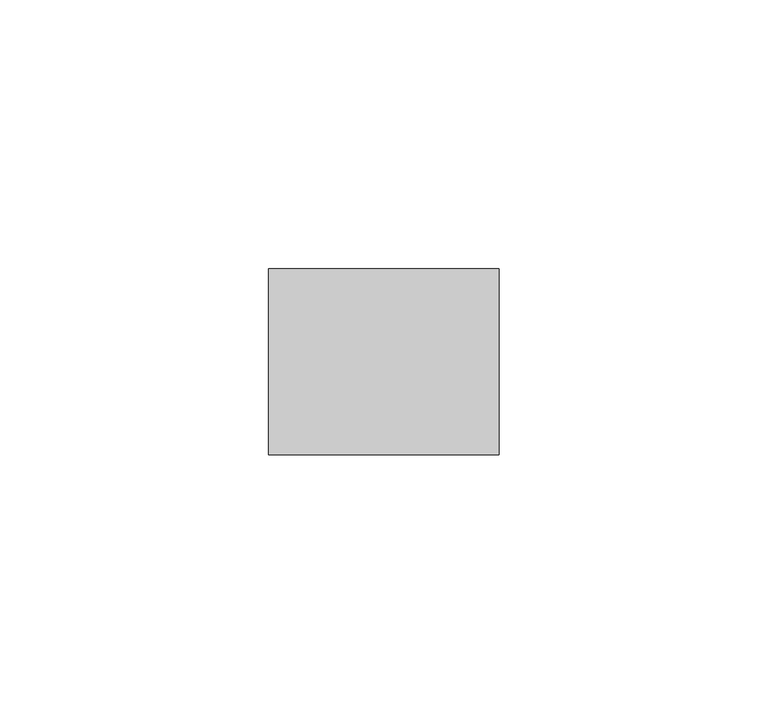
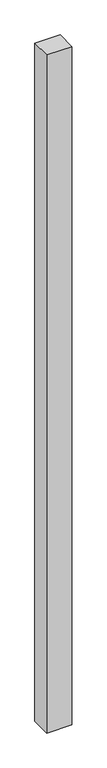
"""IFC4 building model written with IfcOpenShell, lengths in millimetres: proxy geometry, Inner panel:Inner panel:1:Inner panel:1 : Inner panel:Inner panel:300324:300043:Inner panel:1:Inner panel:1 : Inner panel:Inner panel:300324:300043 : Inner panel:Inner panel:1:Inner panel:1 : Inner panel:Inner panel:300324:300043:43 : Inner panel:Inner panel:1:Inner panel:1 : Inner panel:Inner panel:300324:300043:Inner panel:1:Inner panel:1 : Inner panel:Inner panel:300324:300043 : Inner panel:Inner panel:1:Inner panel:1 : Inner panel:Inner panel:300324:300043:300031."""

from ifc_helpers import new_model, si_unit, frame, origin, place, context, project, spatial, polyline, outline, extrude, source, transform, mapped, element, save


def generic_models_e461512d(model_context):
    return source(origin(), model_context, "Body", "SweptSolid", [
        extrude(outline(polyline([(667301.2492239, -568237.7769044), (667344.1117239, -568237.7769044), (667344.1117239, -568272.3525973), (667301.2492239, -568272.3525973), (667301.2492239, -568237.7769044)])), frame((0.0, 0.0, 4946.65), z_axis=(0.0, 0.0, 1.0), x_axis=(1.0, 0.0, 0.0)), (0.0, 0.0, 1.0), 1219.2),
    ])


if __name__ == "__main__":
    model = new_model("IFC4")
    model_context = context("Model", 3, world=origin())
    ifc_project = project(units=[si_unit("LENGTHUNIT", "METRE", prefix="MILLI")], contexts=[model_context])
    site = spatial("IfcSite", under=ifc_project)
    building = spatial("IfcBuilding", under=site)
    placement = place(None, origin())
    generic_models_shape = generic_models_e461512d(model_context)
    element("IfcBuildingElementProxy", 1, Name="Inner panel:Inner panel:1:Inner panel:1 : Inner panel:Inner panel:300324:300043:Inner panel:1:Inner panel:1 : Inner panel:Inner panel:300324:300043 : Inner panel:Inner panel:1:Inner panel:1 : Inner panel:Inner panel:300324:300043:43 : Inner panel:Inner panel:1:Inner panel:1 : Inner panel:Inner panel:300324:300043:Inner panel:1:Inner panel:1 : Inner panel:Inner panel:300324:300043 : Inner panel:Inner panel:1:Inner panel:1 : Inner panel:Inner panel:300324:300043:300031", ObjectType="Inner panel:Inner panel:1:Inner panel:1 : Inner panel:Inner panel:300324:300043:Inner panel:1:Inner panel:1 : Inner panel:Inner panel:300324:300043 : Inner panel:Inner panel:1:Inner panel:1 : Inner panel:Inner panel:300324:300043:43 : Inner panel:Inner panel:1:Inner panel:1 : Inner panel:Inner panel:300324:300043:Inner panel:1:Inner panel:1 : Inner panel:Inner panel:300324:300043 : Inner panel:Inner panel:1:Inner panel:1 : Inner panel:Inner panel:300324:300043:300031", at=placement, inside=building, context=model_context, shape_type="MappedRepresentation", body=[
        mapped(generic_models_shape, transform((0.0, 0.0, 0.0), x_axis=(1.0, 0.0, 0.0), y_axis=(0.0, 1.0, 0.0), z_axis=(0.0, 0.0, 1.0))),
    ])
    save(model, "model.ifc")

# Revit data of these elements
# Type "Inner panel:Inner panel:1:Inner panel:1 : Inner panel:Inner panel:300324:300043:Inner panel:1:Inner panel:1 : Inner panel:Inner panel:300324:300043 : Inner panel:Inner panel:1:Inner panel:1 : Inner panel:Inner panel:300324:300043:43 : Inner panel:Inner panel:1:Inner panel:1 : Inner panel:Inner panel:300324:300043:Inner panel:1:Inner panel:1 : Inner panel:Inner panel:300324:300043 : Inner panel:Inner panel:1:Inner panel:1 : Inner panel:Inner panel:300324:300043:300031"
#   NameOverride = "Inner panel:Inner panel:1:Inner panel:1 : Inner panel:Inner panel:300324:300043:Inner panel:1:Inner panel:1 : Inner panel:Inner panel:300324:300043 : Inner panel:Inner panel:1:Inner panel:1 : Inner panel:Inner panel:300324:300043:300031"
#   ObjectTypeOverride = "Inner panel:1:Inner panel:1 : Inner panel:Inner panel:300324:300043 : Inner panel:Inner panel:1:Inner panel:1 : Inner panel:Inner panel:300324:300043"
#   Reference = "Inner panel"
#   Tag = "300031"
# Element 1 (IfcBuildingElementProxy, "Inner panel:Inner panel:1:Inner panel:1 : Inner panel:Inner panel:300324:300043:Inner panel:1:Inner panel:1 : Inner panel:Inner panel:300324:300043 : Inner panel:Inner panel:1:Inner panel:1 : Inner panel:Inner panel:300324:300043:43 : Inner panel:Inner panel:1:Inner panel:1 : Inner panel:Inner panel:300324:300043:Inner panel:1:Inner panel:1 : Inner panel:Inner panel:300324:300043 : Inner panel:Inner panel:1:Inner panel:1 : Inner panel:Inner panel:300324:300043:300031")
#   Materials on its faces: "BLOCKING - SIZE AS NEC."
# Materials
#   "BLOCKING - SIZE AS NEC.": class "Wood", colour RGB 144 113 62, transparency 0, Description = "Pinus Echinata", Cost = 0
